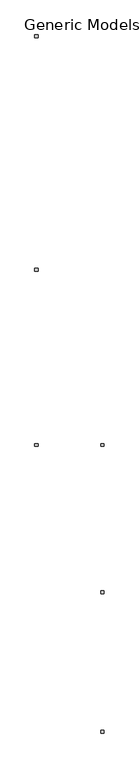
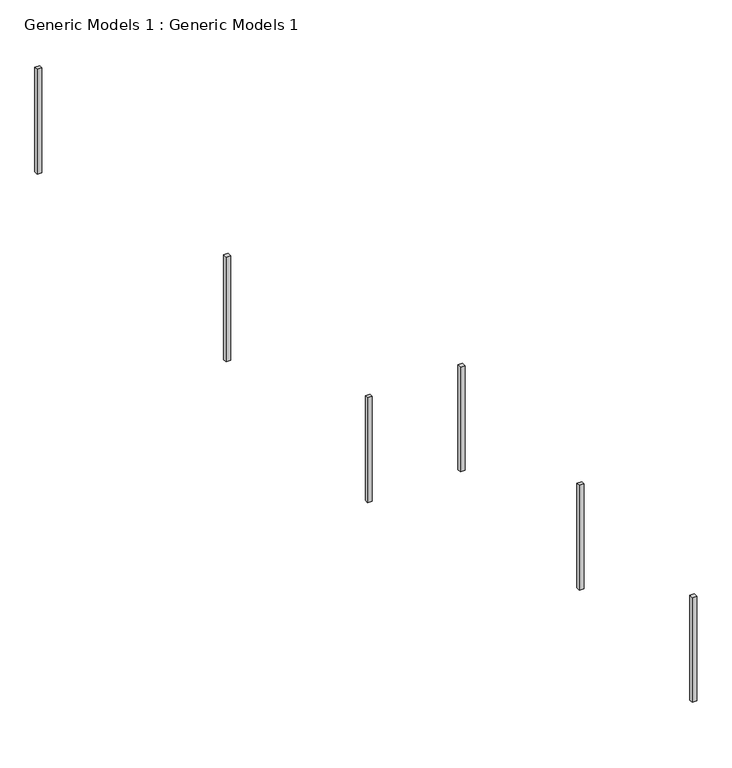
"""IFC4 building model written with IfcOpenShell, lengths in millimetres: proxy geometry, Generic Models 1 : Generic Models 1."""

import ifcopenshell
import ifcopenshell.guid

model = None  # the IFC model being written
_history = None  # IfcOwnerHistory: only IFC2X3 demands one
_inside = {}  # id of a spatial element -> (the spatial element, [elements in it])
_under = {}  # id of a project, library or spatial element -> (it, [spatial elements below it])
_declared = {}  # id of a project -> (the project, [libraries it declares])
_typed = {}  # id of a type object -> (the type object, [elements of that type])
_made_of = {}  # id of a material, layer set ... -> (it, [elements and type objects made of it])


def new_model(schema):
    """Start an empty IFC model of exactly this schema.

    Asked for "IFC4X3", IfcOpenShell would pick the latest addendum, in which some entities
    have other attributes; the version numbers below select the first issue.
    IFC2X3 requires an IfcOwnerHistory on every rooted entity: one is made here for all.
    """
    global model, _history
    if schema == "IFC4X3":
        model = ifcopenshell.file(schema_version=(4, 3, 0, 0))
    else:
        model = ifcopenshell.file(schema=schema)
    _inside.clear()
    _under.clear()
    _declared.clear()
    _typed.clear()
    _made_of.clear()
    _history = None
    if model.schema == "IFC2X3":
        org = make("IfcOrganization", Name="unknown")
        user = make(
            "IfcPersonAndOrganization",
            ThePerson=make("IfcPerson", FamilyName="unknown"),
            TheOrganization=org,
        )
        app = make(
            "IfcApplication",
            ApplicationDeveloper=org,
            Version="unknown",
            ApplicationFullName="unknown",
            ApplicationIdentifier="unknown",
        )
        _history = make(
            "IfcOwnerHistory",
            OwningUser=user,
            OwningApplication=app,
            ChangeAction="ADDED",
            CreationDate=0,
        )
    return model


def make(cls, **values):
    """One entity of the class cls with the attributes given. An attribute that is None is left unset."""
    return model.create_entity(
        cls, **{name: value for name, value in values.items() if value is not None}
    )


def rooted(cls, **values):
    """An entity with a GlobalId (a new one), such as an element, a storey or a relation."""
    return make(cls, GlobalId=ifcopenshell.guid.new(), OwnerHistory=_history, **values)


def si_unit(unit_type, name, prefix=None):
    """IfcSIUnit, for example si_unit("LENGTHUNIT", "METRE", prefix="MILLI")."""
    return make("IfcSIUnit", UnitType=unit_type, Prefix=prefix, Name=name)


def assignment(units):
    """IfcUnitAssignment: the units of a project."""
    return None if units is None else make("IfcUnitAssignment", Units=units)


def point(xyz):
    """IfcCartesianPoint."""
    return None if xyz is None else make("IfcCartesianPoint", Coordinates=xyz)


def direction(xyz):
    """IfcDirection."""
    return None if xyz is None else make("IfcDirection", DirectionRatios=xyz)


def frame(location, z_axis=None, x_axis=None):
    """IfcAxis2Placement3D, a coordinate frame: its origin and axes. An axis left out is left unset."""
    return make(
        "IfcAxis2Placement3D",
        Location=point(location),
        Axis=direction(z_axis),
        RefDirection=direction(x_axis),
    )


def origin():
    """The frame at (0, 0, 0) with its axes left unset."""
    return frame((0.0, 0.0, 0.0))


def place(relative_to, where):
    """IfcLocalPlacement: puts the frame where relative to a parent placement (None: the world)."""
    return make(
        "IfcLocalPlacement", PlacementRelTo=relative_to, RelativePlacement=where
    )


def context(
    kind, dimensions, precision=None, world=None, true_north=None, identifier=None
):
    """IfcGeometricRepresentationContext, for example the 3D "Model" context."""
    return make(
        "IfcGeometricRepresentationContext",
        ContextIdentifier=identifier,
        ContextType=kind,
        CoordinateSpaceDimension=dimensions,
        Precision=precision,
        WorldCoordinateSystem=world,
        TrueNorth=true_north,
    )


def project(units=None, contexts=None):
    """IfcProject with its units and contexts."""
    return rooted(
        "IfcProject",
        Name="project",
        RepresentationContexts=contexts,
        UnitsInContext=assignment(units),
    )


def spatial(cls, under=None, at=None, **own):
    """A site, building, storey or space (cls), placed at a placement, below another one or the project."""
    s = rooted(cls, ObjectPlacement=at, **own)
    if under is not None:
        _under.setdefault(under.id(), (under, []))[1].append(s)
    return s


def polyline(points):
    """IfcPolyline through the points."""
    return make("IfcPolyline", Points=[point(p) for p in points])


def outline(outer, holes=None, kind="AREA"):
    """IfcArbitraryClosedProfileDef: a profile drawn as a closed curve; with holes, ...WithVoids."""
    if holes is None:
        return make("IfcArbitraryClosedProfileDef", ProfileType=kind, OuterCurve=outer)
    return make(
        "IfcArbitraryProfileDefWithVoids",
        ProfileType=kind,
        OuterCurve=outer,
        InnerCurves=holes,
    )


def extrude(swept, where, along, depth):
    """IfcExtrudedAreaSolid: the profile swept, set in the frame where, extruded along a direction by depth."""
    return make(
        "IfcExtrudedAreaSolid",
        SweptArea=swept,
        Position=where,
        ExtrudedDirection=direction(along),
        Depth=depth,
    )


def shape(context_of_items, identifier, shape_type, items):
    """IfcShapeRepresentation: the items that make up one representation, for example the "Body"."""
    return make(
        "IfcShapeRepresentation",
        ContextOfItems=context_of_items,
        RepresentationIdentifier=identifier,
        RepresentationType=shape_type,
        Items=items,
    )


def source(mapping_origin, context_of_items, identifier, shape_type, items):
    """IfcRepresentationMap: a shape defined once, which mapped items show again and again."""
    return make(
        "IfcRepresentationMap",
        MappingOrigin=mapping_origin,
        MappedRepresentation=shape(context_of_items, identifier, shape_type, items),
    )


def transform(
    local_origin,
    x_axis=None,
    y_axis=None,
    z_axis=None,
    scale=None,
    scale2=None,
    scale3=None,
    uniform=True,
):
    """IfcCartesianTransformationOperator3D, or its non-uniform kind. x_axis, y_axis, z_axis: its Axis1, 2, 3."""
    if uniform:
        return make(
            "IfcCartesianTransformationOperator3D",
            Axis1=direction(x_axis),
            Axis2=direction(y_axis),
            LocalOrigin=point(local_origin),
            Scale=scale,
            Axis3=direction(z_axis),
        )
    return make(
        "IfcCartesianTransformationOperator3DnonUniform",
        Axis1=direction(x_axis),
        Axis2=direction(y_axis),
        LocalOrigin=point(local_origin),
        Scale=scale,
        Axis3=direction(z_axis),
        Scale2=scale2,
        Scale3=scale3,
    )


def mapped(mapping_source, mapping_target):
    """IfcMappedItem: shows the shape of a source again, moved by a transform."""
    return make(
        "IfcMappedItem", MappingSource=mapping_source, MappingTarget=mapping_target
    )


def made_of(thing, what):
    """Note that an element or type object is made of a material, layer set ...; save() writes the relation."""
    if what is not None:
        _made_of.setdefault(what.id(), (what, []))[1].append(thing)
    return thing


def element(
    cls,
    number,
    at=None,
    inside=None,
    cuts=None,
    type_object=None,
    material=None,
    context=None,
    identifier="Body",
    shape_type=None,
    held_by="IfcProductDefinitionShape",
    body=None,
    shapes=None,
    **own,
):
    """One element of the class cls, such as IfcWall. Its Tag is "e" and its number.

    at: its placement. inside: the storey or other place that contains it. cuts: it is an
    opening in that element (IfcRelVoidsElement). A single representation is given by context,
    identifier, shape_type and body (its items); several are given by shapes. held_by: the class
    of the entity that holds the representations. save() writes the other relations.
    """
    e = rooted(cls, Tag="e%d" % number, ObjectPlacement=at, **own)
    if body is not None:
        shapes = [shape(context, identifier, shape_type, body)]
    if shapes is not None:
        e.Representation = make(held_by, Representations=shapes)
    if inside is not None:
        _inside.setdefault(inside.id(), (inside, []))[1].append(e)
    if cuts is not None:
        rooted(
            "IfcRelVoidsElement", RelatingBuildingElement=cuts, RelatedOpeningElement=e
        )
    if type_object is not None:
        _typed.setdefault(type_object.id(), (type_object, []))[1].append(e)
    return made_of(e, material)


def aggregate(whole, parts):
    """IfcRelAggregates: a whole, such as a stair, and the parts it consists of."""
    return rooted("IfcRelAggregates", RelatingObject=whole, RelatedObjects=parts)


def save(model, path):
    """Write the relations noted so far, then the file.

    IfcRelAggregates (storeys below a building ...), IfcRelContainedInSpatialStructure (elements
    in a storey), IfcRelDefinesByType, IfcRelAssociatesMaterial and IfcRelDeclares: one each for
    every whole, place, type object, material and project.
    """
    for whole, parts in _under.values():
        aggregate(whole, parts)
    for where, things in _inside.values():
        rooted(
            "IfcRelContainedInSpatialStructure",
            RelatedElements=things,
            RelatingStructure=where,
        )
    for kind, things in _typed.values():
        rooted("IfcRelDefinesByType", RelatedObjects=things, RelatingType=kind)
    for what, things in _made_of.values():
        rooted("IfcRelAssociatesMaterial", RelatedObjects=things, RelatingMaterial=what)
    for by, libraries in _declared.values():
        rooted("IfcRelDeclares", RelatingContext=by, RelatedDefinitions=libraries)
    model.write(path)


def generic_models_1_generic_models_1_90de948b(model_context):
    return source(origin(), model_context, "Body", "SweptSolid", [
        extrude(outline(polyline([(17437.9879668, -9053.7860729), (17407.9879668, -9053.7860729), (17407.9879668, -9028.7860729), (17437.9879668, -9028.7860729), (17437.9879668, -9053.7860729)])), frame((0.0, 0.0, 6858.0), z_axis=(0.0, 0.0, 1.0), x_axis=(1.0, 0.0, 0.0)), (0.0, 0.0, 1.0), 722.1629366),
        extrude(outline(polyline([(17437.9879668, -7778.7860729), (17407.9879668, -7778.7860729), (17407.9879668, -7753.7860729), (17437.9879668, -7753.7860729), (17437.9879668, -7778.7860729)])), frame((0.0, 0.0, 6858.0), z_axis=(0.0, 0.0, 1.0), x_axis=(1.0, 0.0, 0.0)), (0.0, 0.0, 1.0), 722.1629366),
        extrude(outline(polyline([(17437.9879668, -6433.7860729), (17407.9879668, -6433.7860729), (17407.9879668, -6408.7860729), (17437.9879668, -6408.7860729), (17437.9879668, -6433.7860729)])), frame((0.0, 0.0, 6858.0), z_axis=(0.0, 0.0, 1.0), x_axis=(1.0, 0.0, 0.0)), (0.0, 0.0, 1.0), 722.1629366),
        extrude(outline(polyline([(16832.9879668, -6433.7860729), (16802.9879668, -6433.7860729), (16802.9879668, -6408.7860729), (16832.9879668, -6408.7860729), (16832.9879668, -6433.7860729)])), frame((0.0, 0.0, 6858.0), z_axis=(0.0, 0.0, 1.0), x_axis=(1.0, 0.0, 0.0)), (0.0, 0.0, 1.0), 722.1629366),
        extrude(outline(polyline([(16832.9879668, -4833.7860729), (16802.9879668, -4833.7860729), (16802.9879668, -4808.7860729), (16832.9879668, -4808.7860729), (16832.9879668, -4833.7860729)])), frame((0.0, 0.0, 6858.0), z_axis=(0.0, 0.0, 1.0), x_axis=(1.0, 0.0, 0.0)), (0.0, 0.0, 1.0), 722.1629366),
        extrude(outline(polyline([(16832.9879668, -2700.682032), (16802.9879668, -2700.682032), (16802.9879668, -2675.682032), (16832.9879668, -2675.682032), (16832.9879668, -2700.682032)])), frame((0.0, 0.0, 6858.0), z_axis=(0.0, 0.0, 1.0), x_axis=(1.0, 0.0, 0.0)), (0.0, 0.0, 1.0), 722.1629366),
    ])


if __name__ == "__main__":
    model = new_model("IFC4")
    model_context = context("Model", 3, world=origin())
    ifc_project = project(units=[si_unit("LENGTHUNIT", "METRE", prefix="MILLI")], contexts=[model_context])
    site = spatial("IfcSite", under=ifc_project)
    building = spatial("IfcBuilding", under=site)
    placement = place(None, origin())
    generic_models_1_generic_models_1_shape = generic_models_1_generic_models_1_90de948b(model_context)
    element("IfcBuildingElementProxy", 1, Name="Generic Models 1 : Generic Models 1", ObjectType="Generic Models 1 : Generic Models 1", at=placement, inside=building, context=model_context, shape_type="MappedRepresentation", body=[
        mapped(generic_models_1_generic_models_1_shape, transform((0.0, 0.0, 0.0), x_axis=(1.0, 0.0, 0.0), y_axis=(0.0, 1.0, 0.0), z_axis=(0.0, 0.0, 1.0))),
    ])
    save(model, "model.ifc")

# Revit data of these elements
# Element 1 (IfcBuildingElementProxy, "Generic Models 1 : Generic Models 1")
#   Materials on its faces: "METAL TEXTURE"
# Materials
#   "METAL TEXTURE": class "Generic", colour RGB 120 120 120, transparency 0, Cost = 0
